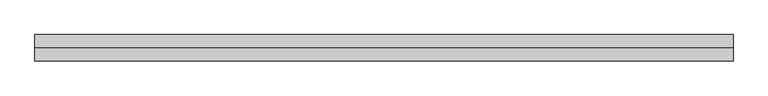
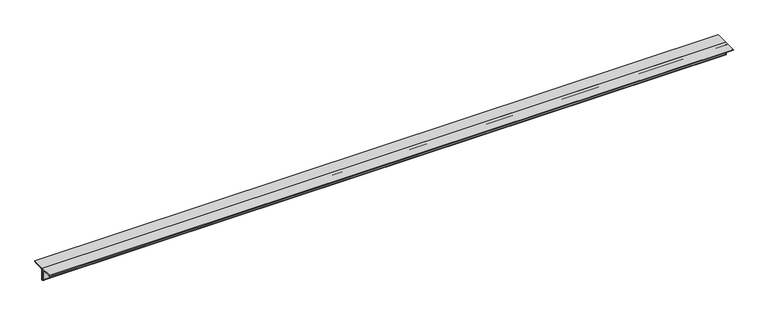
"""IFC4 building model written with IfcOpenShell, lengths in millimetres: member geometry, Steel Framing_2Ls_KS : H_SB_AR_S02_2Ls-100x100x10_VBR1."""

from ifc_helpers import new_model, si_unit, point, frame, frame_2d, origin, place, context, project, spatial, polyline, circle_curve, trimmed, segment, composite_curve, outline, extrude, source, transform, mapped, element, save


def member_0930e643(model_context):
    return source(origin(), model_context, "Body", "SweptSolid", [
        extrude(outline(composite_curve([segment(polyline([(0.0, 28.2), (0.0, -71.8)]), True, "CONTINUOUS"), segment(trimmed(circle_curve(frame_2d((0.0, -61.8)), 10.0), [point((0.0, -71.8))], [point((-10.0, -61.8))], False, "CARTESIAN"), True, "CONTINUOUS"), segment(polyline([(-10.0, -61.8), (-10.0, 8.2)]), True, "CONTINUOUS"), segment(trimmed(circle_curve(frame_2d((-20.0, 8.2)), 10.0), [point((-10.0, 8.2))], [point((-20.0, 18.2))], True, "CARTESIAN"), True, "CONTINUOUS"), segment(polyline([(-20.0, 18.2), (-90.0, 18.2)]), True, "CONTINUOUS"), segment(trimmed(circle_curve(frame_2d((-90.0, 28.2)), 10.0), [point((-90.0, 18.2))], [point((-100.0, 28.2))], False, "CARTESIAN"), True, "CONTINUOUS"), segment(polyline([(-100.0, 28.2), (0.0, 28.2)]), True, "CONTINUOUS")], self_intersect=False)), frame((-2711.0698468, 0.0, 0.0), z_axis=(1.0, 0.0, 0.0), x_axis=(0.0, 1.0, 0.0)), (0.0, 0.0, 1.0), 5293.9751588),
        extrude(outline(composite_curve([segment(polyline([(0.0, 28.2), (100.0, 28.2)]), True, "CONTINUOUS"), segment(trimmed(circle_curve(frame_2d((90.0, 28.2)), 10.0), [point((100.0, 28.2))], [point((90.0, 18.2))], False, "CARTESIAN"), True, "CONTINUOUS"), segment(polyline([(90.0, 18.2), (20.0, 18.2)]), True, "CONTINUOUS"), segment(trimmed(circle_curve(frame_2d((20.0, 8.2)), 10.0), [point((20.0, 18.2))], [point((10.0, 8.2))], True, "CARTESIAN"), True, "CONTINUOUS"), segment(polyline([(10.0, 8.2), (10.0, -61.8)]), True, "CONTINUOUS"), segment(trimmed(circle_curve(frame_2d((0.0, -61.8)), 10.0), [point((10.0, -61.8))], [point((0.0, -71.8))], False, "CARTESIAN"), True, "CONTINUOUS"), segment(polyline([(0.0, -71.8), (0.0, 28.2)]), True, "CONTINUOUS")], self_intersect=False)), frame((-2711.0698468, 0.0, 0.0), z_axis=(1.0, 0.0, 0.0), x_axis=(0.0, 1.0, 0.0)), (0.0, 0.0, 1.0), 5293.9751588),
    ])


if __name__ == "__main__":
    model = new_model("IFC4")
    model_context = context("Model", 3, world=origin())
    ifc_project = project(units=[si_unit("LENGTHUNIT", "METRE", prefix="MILLI")], contexts=[model_context])
    site = spatial("IfcSite", under=ifc_project)
    building = spatial("IfcBuilding", under=site)
    placement = place(None, origin())
    member_shape = member_0930e643(model_context)
    element("IfcMember", 1, ObjectType="Steel Framing_2Ls_KS : H_SB_AR_S02_2Ls-100x100x10_VBR1", at=placement, inside=building, context=model_context, shape_type="MappedRepresentation", body=[
        mapped(member_shape, transform((0.0, 0.0, 0.0), x_axis=(1.0, 0.0, 0.0), y_axis=(0.0, 1.0, 0.0), z_axis=(0.0, 0.0, 1.0))),
    ])
    save(model, "model.ifc")

# Revit data of these elements
# Type "Steel Framing_2Ls_KS : H_SB_AR_S02_2Ls-100x100x10_VBR1"
#   Type Comments = "MAIN"
#   Type Mark = "VBR1"
#   H_SectionID = "2Ls-100x100x10"
#   Assembly Code = "B10"
#   Legs = "LLBB"
#   H_Ratio for Additional Steel Plate = 0.2
#   W = 0
#   Perimeter = 0.80 m²/m
#   Nominal Weight = 29.80 kgf/m
#   Length [instance default] = 1524 mm
#   Space = 0 mm
#   b = 100 mm
#   d = 100 mm
#   t = 10 mm
#   y = 28.2 mm
#   A = 0.0038 m²
#   Structural Material [instance default] = Steel, 45-345
# Element 1 (IfcMember, "Steel Framing_2Ls_KS : H_SB_AR_S02_2Ls-100x100x10_VBR1")
#   Materials on its faces: "Steel, 45-345"
# Materials
#   "Steel, 45-345": class "Metal", colour RGB 189 187 185, transparency 0, Description = "Steel 345 MPa", Cost = 0
